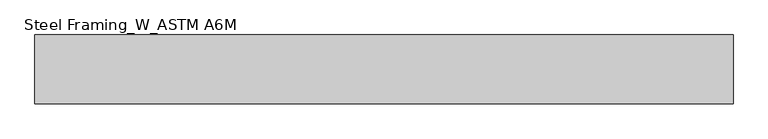
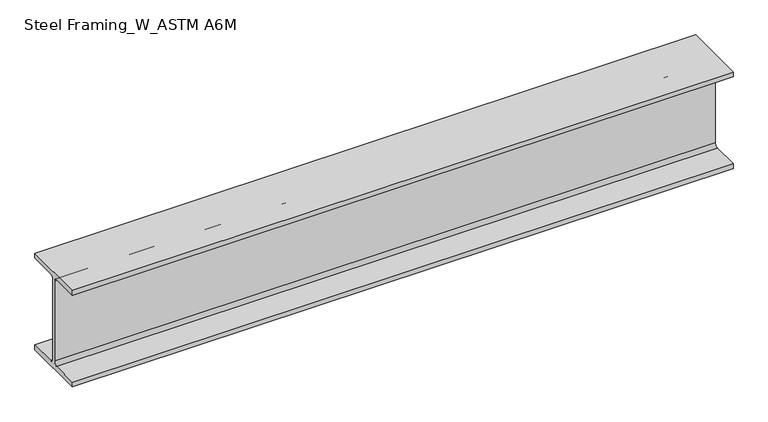
"""IFC4 building model written with IfcOpenShell, lengths in millimetres: beam geometry, Steel Framing_W_ASTM A6M : H_SB_AR_S02_W200x31.3_B6."""

import ifcopenshell
import ifcopenshell.guid

model = None  # the IFC model being written
_history = None  # IfcOwnerHistory: only IFC2X3 demands one
_inside = {}  # id of a spatial element -> (the spatial element, [elements in it])
_under = {}  # id of a project, library or spatial element -> (it, [spatial elements below it])
_declared = {}  # id of a project -> (the project, [libraries it declares])
_typed = {}  # id of a type object -> (the type object, [elements of that type])
_made_of = {}  # id of a material, layer set ... -> (it, [elements and type objects made of it])


def new_model(schema):
    """Start an empty IFC model of exactly this schema.

    Asked for "IFC4X3", IfcOpenShell would pick the latest addendum, in which some entities
    have other attributes; the version numbers below select the first issue.
    IFC2X3 requires an IfcOwnerHistory on every rooted entity: one is made here for all.
    """
    global model, _history
    if schema == "IFC4X3":
        model = ifcopenshell.file(schema_version=(4, 3, 0, 0))
    else:
        model = ifcopenshell.file(schema=schema)
    _inside.clear()
    _under.clear()
    _declared.clear()
    _typed.clear()
    _made_of.clear()
    _history = None
    if model.schema == "IFC2X3":
        org = make("IfcOrganization", Name="unknown")
        user = make(
            "IfcPersonAndOrganization",
            ThePerson=make("IfcPerson", FamilyName="unknown"),
            TheOrganization=org,
        )
        app = make(
            "IfcApplication",
            ApplicationDeveloper=org,
            Version="unknown",
            ApplicationFullName="unknown",
            ApplicationIdentifier="unknown",
        )
        _history = make(
            "IfcOwnerHistory",
            OwningUser=user,
            OwningApplication=app,
            ChangeAction="ADDED",
            CreationDate=0,
        )
    return model


def make(cls, **values):
    """One entity of the class cls with the attributes given. An attribute that is None is left unset."""
    return model.create_entity(
        cls, **{name: value for name, value in values.items() if value is not None}
    )


def rooted(cls, **values):
    """An entity with a GlobalId (a new one), such as an element, a storey or a relation."""
    return make(cls, GlobalId=ifcopenshell.guid.new(), OwnerHistory=_history, **values)


def si_unit(unit_type, name, prefix=None):
    """IfcSIUnit, for example si_unit("LENGTHUNIT", "METRE", prefix="MILLI")."""
    return make("IfcSIUnit", UnitType=unit_type, Prefix=prefix, Name=name)


def assignment(units):
    """IfcUnitAssignment: the units of a project."""
    return None if units is None else make("IfcUnitAssignment", Units=units)


def point(xyz):
    """IfcCartesianPoint."""
    return None if xyz is None else make("IfcCartesianPoint", Coordinates=xyz)


def direction(xyz):
    """IfcDirection."""
    return None if xyz is None else make("IfcDirection", DirectionRatios=xyz)


def frame(location, z_axis=None, x_axis=None):
    """IfcAxis2Placement3D, a coordinate frame: its origin and axes. An axis left out is left unset."""
    return make(
        "IfcAxis2Placement3D",
        Location=point(location),
        Axis=direction(z_axis),
        RefDirection=direction(x_axis),
    )


def frame_2d(location, x_axis=None):
    """IfcAxis2Placement2D, a coordinate frame in the plane: its origin and x axis."""
    return make(
        "IfcAxis2Placement2D", Location=point(location), RefDirection=direction(x_axis)
    )


def origin():
    """The frame at (0, 0, 0) with its axes left unset."""
    return frame((0.0, 0.0, 0.0))


def place(relative_to, where):
    """IfcLocalPlacement: puts the frame where relative to a parent placement (None: the world)."""
    return make(
        "IfcLocalPlacement", PlacementRelTo=relative_to, RelativePlacement=where
    )


def context(
    kind, dimensions, precision=None, world=None, true_north=None, identifier=None
):
    """IfcGeometricRepresentationContext, for example the 3D "Model" context."""
    return make(
        "IfcGeometricRepresentationContext",
        ContextIdentifier=identifier,
        ContextType=kind,
        CoordinateSpaceDimension=dimensions,
        Precision=precision,
        WorldCoordinateSystem=world,
        TrueNorth=true_north,
    )


def project(units=None, contexts=None):
    """IfcProject with its units and contexts."""
    return rooted(
        "IfcProject",
        Name="project",
        RepresentationContexts=contexts,
        UnitsInContext=assignment(units),
    )


def spatial(cls, under=None, at=None, **own):
    """A site, building, storey or space (cls), placed at a placement, below another one or the project."""
    s = rooted(cls, ObjectPlacement=at, **own)
    if under is not None:
        _under.setdefault(under.id(), (under, []))[1].append(s)
    return s


def polyline(points):
    """IfcPolyline through the points."""
    return make("IfcPolyline", Points=[point(p) for p in points])


def circle_curve(where, radius):
    """IfcCircle in the frame where."""
    return make("IfcCircle", Position=where, Radius=radius)


def trimmed(basis, trim1, trim2, sense, master):
    """IfcTrimmedCurve: the piece of a basis curve between two trims."""
    return make(
        "IfcTrimmedCurve",
        BasisCurve=basis,
        Trim1=trim1,
        Trim2=trim2,
        SenseAgreement=sense,
        MasterRepresentation=master,
    )


def segment(curve, same_sense, transition):
    """IfcCompositeCurveSegment."""
    return make(
        "IfcCompositeCurveSegment",
        Transition=transition,
        SameSense=same_sense,
        ParentCurve=curve,
    )


def composite_curve(segments, self_intersect=None):
    """IfcCompositeCurve: segments joined end to end."""
    return make("IfcCompositeCurve", Segments=segments, SelfIntersect=self_intersect)


def outline(outer, holes=None, kind="AREA"):
    """IfcArbitraryClosedProfileDef: a profile drawn as a closed curve; with holes, ...WithVoids."""
    if holes is None:
        return make("IfcArbitraryClosedProfileDef", ProfileType=kind, OuterCurve=outer)
    return make(
        "IfcArbitraryProfileDefWithVoids",
        ProfileType=kind,
        OuterCurve=outer,
        InnerCurves=holes,
    )


def extrude(swept, where, along, depth):
    """IfcExtrudedAreaSolid: the profile swept, set in the frame where, extruded along a direction by depth."""
    return make(
        "IfcExtrudedAreaSolid",
        SweptArea=swept,
        Position=where,
        ExtrudedDirection=direction(along),
        Depth=depth,
    )


def shape(context_of_items, identifier, shape_type, items):
    """IfcShapeRepresentation: the items that make up one representation, for example the "Body"."""
    return make(
        "IfcShapeRepresentation",
        ContextOfItems=context_of_items,
        RepresentationIdentifier=identifier,
        RepresentationType=shape_type,
        Items=items,
    )


def source(mapping_origin, context_of_items, identifier, shape_type, items):
    """IfcRepresentationMap: a shape defined once, which mapped items show again and again."""
    return make(
        "IfcRepresentationMap",
        MappingOrigin=mapping_origin,
        MappedRepresentation=shape(context_of_items, identifier, shape_type, items),
    )


def transform(
    local_origin,
    x_axis=None,
    y_axis=None,
    z_axis=None,
    scale=None,
    scale2=None,
    scale3=None,
    uniform=True,
):
    """IfcCartesianTransformationOperator3D, or its non-uniform kind. x_axis, y_axis, z_axis: its Axis1, 2, 3."""
    if uniform:
        return make(
            "IfcCartesianTransformationOperator3D",
            Axis1=direction(x_axis),
            Axis2=direction(y_axis),
            LocalOrigin=point(local_origin),
            Scale=scale,
            Axis3=direction(z_axis),
        )
    return make(
        "IfcCartesianTransformationOperator3DnonUniform",
        Axis1=direction(x_axis),
        Axis2=direction(y_axis),
        LocalOrigin=point(local_origin),
        Scale=scale,
        Axis3=direction(z_axis),
        Scale2=scale2,
        Scale3=scale3,
    )


def mapped(mapping_source, mapping_target):
    """IfcMappedItem: shows the shape of a source again, moved by a transform."""
    return make(
        "IfcMappedItem", MappingSource=mapping_source, MappingTarget=mapping_target
    )


def made_of(thing, what):
    """Note that an element or type object is made of a material, layer set ...; save() writes the relation."""
    if what is not None:
        _made_of.setdefault(what.id(), (what, []))[1].append(thing)
    return thing


def element(
    cls,
    number,
    at=None,
    inside=None,
    cuts=None,
    type_object=None,
    material=None,
    context=None,
    identifier="Body",
    shape_type=None,
    held_by="IfcProductDefinitionShape",
    body=None,
    shapes=None,
    **own,
):
    """One element of the class cls, such as IfcWall. Its Tag is "e" and its number.

    at: its placement. inside: the storey or other place that contains it. cuts: it is an
    opening in that element (IfcRelVoidsElement). A single representation is given by context,
    identifier, shape_type and body (its items); several are given by shapes. held_by: the class
    of the entity that holds the representations. save() writes the other relations.
    """
    e = rooted(cls, Tag="e%d" % number, ObjectPlacement=at, **own)
    if body is not None:
        shapes = [shape(context, identifier, shape_type, body)]
    if shapes is not None:
        e.Representation = make(held_by, Representations=shapes)
    if inside is not None:
        _inside.setdefault(inside.id(), (inside, []))[1].append(e)
    if cuts is not None:
        rooted(
            "IfcRelVoidsElement", RelatingBuildingElement=cuts, RelatedOpeningElement=e
        )
    if type_object is not None:
        _typed.setdefault(type_object.id(), (type_object, []))[1].append(e)
    return made_of(e, material)


def aggregate(whole, parts):
    """IfcRelAggregates: a whole, such as a stair, and the parts it consists of."""
    return rooted("IfcRelAggregates", RelatingObject=whole, RelatedObjects=parts)


def save(model, path):
    """Write the relations noted so far, then the file.

    IfcRelAggregates (storeys below a building ...), IfcRelContainedInSpatialStructure (elements
    in a storey), IfcRelDefinesByType, IfcRelAssociatesMaterial and IfcRelDeclares: one each for
    every whole, place, type object, material and project.
    """
    for whole, parts in _under.values():
        aggregate(whole, parts)
    for where, things in _inside.values():
        rooted(
            "IfcRelContainedInSpatialStructure",
            RelatedElements=things,
            RelatingStructure=where,
        )
    for kind, things in _typed.values():
        rooted("IfcRelDefinesByType", RelatedObjects=things, RelatingType=kind)
    for what, things in _made_of.values():
        rooted("IfcRelAssociatesMaterial", RelatedObjects=things, RelatingMaterial=what)
    for by, libraries in _declared.values():
        rooted("IfcRelDeclares", RelatingContext=by, RelatedDefinitions=libraries)
    model.write(path)


def steel_framing_w_astm_a6m_e50dfa28(model_context):
    return source(origin(), model_context, "Body", "SweptSolid", [
        extrude(outline(composite_curve([segment(polyline([(67.0, -94.8), (67.0, -105.0), (-67.0, -105.0), (-67.0, -94.8), (-10.775, -94.8)]), True, "CONTINUOUS"), segment(trimmed(circle_curve(frame_2d((-10.775, -87.2)), 7.6), [point((-10.775, -94.8))], [point((-3.175, -87.2))], True, "CARTESIAN"), True, "CONTINUOUS"), segment(polyline([(-3.175, -87.2), (-3.175, 87.2)]), True, "CONTINUOUS"), segment(trimmed(circle_curve(frame_2d((-10.775, 87.2)), 7.6), [point((-3.175, 87.2))], [point((-10.775, 94.8))], True, "CARTESIAN"), True, "CONTINUOUS"), segment(polyline([(-10.775, 94.8), (-67.0, 94.8), (-67.0, 105.0), (67.0, 105.0), (67.0, 94.8), (10.775, 94.8)]), True, "CONTINUOUS"), segment(trimmed(circle_curve(frame_2d((10.775, 87.2)), 7.6), [point((10.775, 94.8))], [point((3.175, 87.2))], True, "CARTESIAN"), True, "CONTINUOUS"), segment(polyline([(3.175, 87.2), (3.175, -87.2)]), True, "CONTINUOUS"), segment(trimmed(circle_curve(frame_2d((10.775, -87.2)), 7.6), [point((3.175, -87.2))], [point((10.775, -94.8))], True, "CARTESIAN"), True, "CONTINUOUS"), segment(polyline([(10.775, -94.8), (67.0, -94.8)]), True, "CONTINUOUS")], self_intersect=False)), frame((-660.3, 0.0, 0.0), z_axis=(1.0, 0.0, 0.0), x_axis=(0.0, 1.0, 0.0)), (0.0, 0.0, 1.0), 1362.1),
    ])


if __name__ == "__main__":
    model = new_model("IFC4")
    model_context = context("Model", 3, world=origin())
    ifc_project = project(units=[si_unit("LENGTHUNIT", "METRE", prefix="MILLI")], contexts=[model_context])
    site = spatial("IfcSite", under=ifc_project)
    building = spatial("IfcBuilding", under=site)
    placement = place(None, origin())
    steel_framing_w_astm_a6m_shape = steel_framing_w_astm_a6m_e50dfa28(model_context)
    element("IfcBeam", 1, ObjectType="Steel Framing_W_ASTM A6M : H_SB_AR_S02_W200x31.3_B6", at=placement, inside=building, context=model_context, shape_type="MappedRepresentation", body=[
        mapped(steel_framing_w_astm_a6m_shape, transform((0.0, 0.0, 0.0), x_axis=(1.0, 0.0, 0.0), y_axis=(0.0, 1.0, 0.0), z_axis=(0.0, 0.0, 1.0))),
    ])
    save(model, "model.ifc")

# Revit data of these elements
# Type "Steel Framing_W_ASTM A6M : H_SB_AR_S02_W200x31.3_B6"
#   Type Mark = "B6"
#   Section Name Key = "W8x21"
#   Width = 13.4 cm
#   Web Thickness = 0.635 cm
#   Web Fillet = 0.76 cm
#   Warping Constant = 40800.0 cm⁶
#   Torsional Moment of Inertia = 11.70 cm⁴
#   Section Area = 39.7 cm²
#   Plastic Modulus weak axis = 93.2 cm³
#   Plastic Modulus strong axis = 334.0 cm³
#   Perimeter = 0.93 m²/m
#   Nominal Weight = 31.30 kgf/m
#   Moment of Inertia weak axis = 407.00 cm⁴
#   Moment of Inertia strong axis = 3130.00 cm⁴
#   Height = 21.0 cm
#   Flange Thickness = 1.02 cm
#   Elastic Modulus weak axis = 60.8 cm³
#   Elastic Modulus strong axis = 298.0 cm³
#   Centroid Vertical = 10.5 cm
#   Centroid Horizontal = 6.7 cm
#   Length [instance default] = 1500 mm
#   Structural Material [instance default] = Steel, 45-345
#   Bolt Spacing = 0
#   Assembly Code = ""
# Element 1 (IfcBeam, "Steel Framing_W_ASTM A6M : H_SB_AR_S02_W200x31.3_B6")
#   Materials on its faces: "Steel, 45-345"
# Materials
#   "Steel, 45-345": class "Metal", colour RGB 189 187 185, transparency 0, Description = "Steel 345 MPa", Cost = 0
